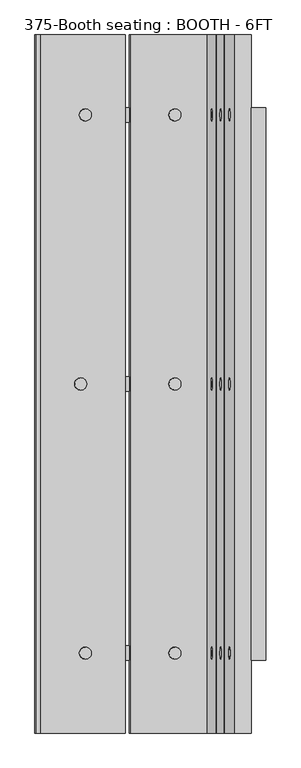
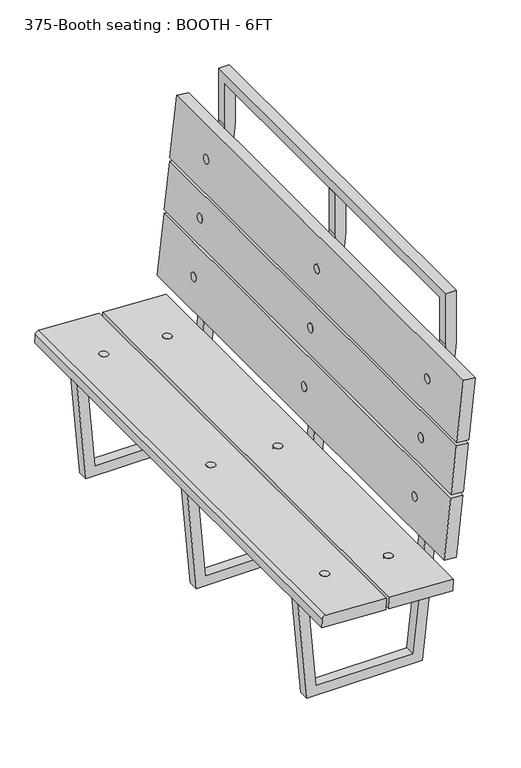
"""IFC4 building model written with IfcOpenShell, lengths in millimetres: furniture geometry, 375-Booth seating : BOOTH - 6FT."""

from ifc_helpers import new_model, si_unit, point, frame, frame_2d, origin, place, context, project, spatial, polyline, circle_curve, trimmed, segment, composite_curve, outline, extrude, faceted_brep, source, transform, mapped, element, save


def furniture_375_booth_seating_booth_6ft_239d0368(model_context):
    return source(origin(), model_context, "Body", "SolidModel", [
        extrude(outline(composite_curve([segment(trimmed(circle_curve(frame_2d((0.0, 15.875)), 15.875), [point((0.0, 31.75))], [point((0.0, 0.0))], False, "CARTESIAN"), True, "CONTINUOUS"), segment(trimmed(circle_curve(frame_2d((0.0, 15.875)), 15.875), [point((0.0, 0.0))], [point((0.0, 31.75))], False, "CARTESIAN"), True, "CONTINUOUS")], self_intersect=False)), frame((476.8022404, -688.975, 403.0070028), z_axis=(0.052335956242943765, 0.0, 0.9986295347545739), x_axis=(-0.9986295347545739, 0.0, 0.052335956242943765)), (0.0, 0.0, 1.0), 44.45),
        extrude(outline(composite_curve([segment(trimmed(circle_curve(frame_2d((-234.95, 15.875)), 15.875), [point((-234.95, 31.75))], [point((-234.95, 0.0))], False, "CARTESIAN"), True, "CONTINUOUS"), segment(trimmed(circle_curve(frame_2d((-234.95, 15.875)), 15.875), [point((-234.95, 0.0))], [point((-234.95, 31.75))], False, "CARTESIAN"), True, "CONTINUOUS")], self_intersect=False)), frame((476.8022404, -688.975, 403.0070028), z_axis=(0.052335956242943765, 0.0, 0.9986295347545739), x_axis=(-0.9986295347545739, 0.0, 0.052335956242943765)), (0.0, 0.0, 1.0), 44.45),
        extrude(outline(composite_curve([segment(trimmed(circle_curve(frame_2d((0.0, -1393.825)), 15.875), [point((0.0, -1377.95))], [point((0.0, -1409.7))], False, "CARTESIAN"), True, "CONTINUOUS"), segment(trimmed(circle_curve(frame_2d((0.0, -1393.825)), 15.875), [point((0.0, -1409.7))], [point((0.0, -1377.95))], False, "CARTESIAN"), True, "CONTINUOUS")], self_intersect=False)), frame((476.8022404, -688.975, 403.0070028), z_axis=(0.052335956242943765, 0.0, 0.9986295347545739), x_axis=(-0.9986295347545739, 0.0, 0.052335956242943765)), (0.0, 0.0, 1.0), 44.45),
        extrude(outline(composite_curve([segment(trimmed(circle_curve(frame_2d((-234.95, -1393.825)), 15.875), [point((-234.95, -1377.95))], [point((-234.95, -1409.7))], False, "CARTESIAN"), True, "CONTINUOUS"), segment(trimmed(circle_curve(frame_2d((-234.95, -1393.825)), 15.875), [point((-234.95, -1409.7))], [point((-234.95, -1377.95))], False, "CARTESIAN"), True, "CONTINUOUS")], self_intersect=False)), frame((476.8022404, -688.975, 403.0070028), z_axis=(0.052335956242943765, 0.0, 0.9986295347545739), x_axis=(-0.9986295347545739, 0.0, 0.052335956242943765)), (0.0, 0.0, 1.0), 44.45),
        extrude(outline(composite_curve([segment(trimmed(circle_curve(frame_2d((0.0, 15.875)), 15.875), [point((0.0, 31.75))], [point((0.0, 0.0))], False, "CARTESIAN"), True, "CONTINUOUS"), segment(trimmed(circle_curve(frame_2d((0.0, 15.875)), 15.875), [point((0.0, 0.0))], [point((0.0, 31.75))], False, "CARTESIAN"), True, "CONTINUOUS")], self_intersect=False)), frame((900.6975371, 720.725, 1069.1522612), z_axis=(-0.9945218953682735, 0.0, 0.10452846326765225), x_axis=(-0.10452846326765225, 0.0, -0.9945218953682735)), (0.0, 0.0, 1.0), 44.45),
        extrude(outline(composite_curve([segment(trimmed(circle_curve(frame_2d((222.2499999, 15.875)), 15.875), [point((222.2499999, 31.75))], [point((222.2499999, 0.0))], False, "CARTESIAN"), True, "CONTINUOUS"), segment(trimmed(circle_curve(frame_2d((222.2499999, 15.875)), 15.875), [point((222.2499999, 0.0))], [point((222.2499999, 31.75))], False, "CARTESIAN"), True, "CONTINUOUS")], self_intersect=False)), frame((900.6975371, 720.725, 1069.1522612), z_axis=(-0.9945218953682735, 0.0, 0.10452846326765225), x_axis=(-0.10452846326765225, 0.0, -0.9945218953682735)), (0.0, 0.0, 1.0), 44.45),
        extrude(outline(composite_curve([segment(trimmed(circle_curve(frame_2d((444.5, 15.875)), 15.875), [point((444.5, 31.75))], [point((444.5, 0.0))], False, "CARTESIAN"), True, "CONTINUOUS"), segment(trimmed(circle_curve(frame_2d((444.5, 15.875)), 15.875), [point((444.5, 0.0))], [point((444.5, 31.75))], False, "CARTESIAN"), True, "CONTINUOUS")], self_intersect=False)), frame((900.6975371, 720.725, 1069.1522612), z_axis=(-0.9945218953682735, 0.0, 0.10452846326765225), x_axis=(-0.10452846326765225, 0.0, -0.9945218953682735)), (0.0, 0.0, 1.0), 44.45),
        extrude(outline(composite_curve([segment(trimmed(circle_curve(frame_2d((0.0, 1425.575)), 15.875), [point((0.0, 1441.45))], [point((0.0, 1409.7))], False, "CARTESIAN"), True, "CONTINUOUS"), segment(trimmed(circle_curve(frame_2d((0.0, 1425.575)), 15.875), [point((0.0, 1409.7))], [point((0.0, 1441.45))], False, "CARTESIAN"), True, "CONTINUOUS")], self_intersect=False)), frame((900.6975371, 720.725, 1069.1522612), z_axis=(-0.9945218953682735, 0.0, 0.10452846326765225), x_axis=(-0.10452846326765225, 0.0, -0.9945218953682735)), (0.0, 0.0, 1.0), 44.45),
        extrude(outline(composite_curve([segment(trimmed(circle_curve(frame_2d((222.2499999, 1425.575)), 15.875), [point((222.2499999, 1441.45))], [point((222.2499999, 1409.7))], False, "CARTESIAN"), True, "CONTINUOUS"), segment(trimmed(circle_curve(frame_2d((222.2499999, 1425.575)), 15.875), [point((222.2499999, 1409.7))], [point((222.2499999, 1441.45))], False, "CARTESIAN"), True, "CONTINUOUS")], self_intersect=False)), frame((900.6975371, 720.725, 1069.1522612), z_axis=(-0.9945218953682735, 0.0, 0.10452846326765225), x_axis=(-0.10452846326765225, 0.0, -0.9945218953682735)), (0.0, 0.0, 1.0), 44.45),
        extrude(outline(composite_curve([segment(trimmed(circle_curve(frame_2d((444.5, 1425.575)), 15.875), [point((444.5, 1441.45))], [point((444.5, 1409.7))], False, "CARTESIAN"), True, "CONTINUOUS"), segment(trimmed(circle_curve(frame_2d((444.5, 1425.575)), 15.875), [point((444.5, 1409.7))], [point((444.5, 1441.45))], False, "CARTESIAN"), True, "CONTINUOUS")], self_intersect=False)), frame((900.6975371, 720.725, 1069.1522612), z_axis=(-0.9945218953682735, 0.0, 0.10452846326765225), x_axis=(-0.10452846326765225, 0.0, -0.9945218953682735)), (0.0, 0.0, 1.0), 44.45),
        extrude(outline(composite_curve([segment(trimmed(circle_curve(frame_2d((0.0, 15.875)), 15.875), [point((0.0, 31.75))], [point((0.0, 0.0))], False, "CARTESIAN"), True, "CONTINUOUS"), segment(trimmed(circle_curve(frame_2d((0.0, 15.875)), 15.875), [point((0.0, 0.0))], [point((0.0, 31.75))], False, "CARTESIAN"), True, "CONTINUOUS")], self_intersect=False)), frame((464.1196453, 15.875, 403.6716695), z_axis=(0.052335956242943765, 0.0, 0.9986295347545739), x_axis=(-0.9986295347545739, 0.0, 0.052335956242943765)), (0.0, 0.0, 1.0), 44.45),
        extrude(outline(composite_curve([segment(trimmed(circle_curve(frame_2d((-247.65, 15.875)), 15.875), [point((-247.65, 31.75))], [point((-247.65, 0.0))], False, "CARTESIAN"), True, "CONTINUOUS"), segment(trimmed(circle_curve(frame_2d((-247.65, 15.875)), 15.875), [point((-247.65, 0.0))], [point((-247.65, 31.75))], False, "CARTESIAN"), True, "CONTINUOUS")], self_intersect=False)), frame((464.1196453, 15.875, 403.6716695), z_axis=(0.052335956242943765, 0.0, 0.9986295347545739), x_axis=(-0.9986295347545739, 0.0, 0.052335956242943765)), (0.0, 0.0, 1.0), 44.45),
        extrude(outline(composite_curve([segment(trimmed(circle_curve(frame_2d((0.0, 15.875)), 15.875), [point((0.0, 31.75))], [point((0.0, 0.0))], False, "CARTESIAN"), True, "CONTINUOUS"), segment(trimmed(circle_curve(frame_2d((0.0, 15.875)), 15.875), [point((0.0, 0.0))], [point((0.0, 31.75))], False, "CARTESIAN"), True, "CONTINUOUS")], self_intersect=False)), frame((900.6975371, 15.875, 1069.1522612), z_axis=(-0.9945218953682735, 0.0, 0.10452846326765225), x_axis=(-0.10452846326765225, 0.0, -0.9945218953682735)), (0.0, 0.0, 1.0), 44.45),
        extrude(outline(composite_curve([segment(trimmed(circle_curve(frame_2d((222.2499999, 15.875)), 15.875), [point((222.2499999, 31.75))], [point((222.2499999, 0.0))], False, "CARTESIAN"), True, "CONTINUOUS"), segment(trimmed(circle_curve(frame_2d((222.2499999, 15.875)), 15.875), [point((222.2499999, 0.0))], [point((222.2499999, 31.75))], False, "CARTESIAN"), True, "CONTINUOUS")], self_intersect=False)), frame((900.6975371, 15.875, 1069.1522612), z_axis=(-0.9945218953682735, 0.0, 0.10452846326765225), x_axis=(-0.10452846326765225, 0.0, -0.9945218953682735)), (0.0, 0.0, 1.0), 44.45),
        extrude(outline(composite_curve([segment(trimmed(circle_curve(frame_2d((444.5, 15.875)), 15.875), [point((444.5, 31.75))], [point((444.5, 0.0))], False, "CARTESIAN"), True, "CONTINUOUS"), segment(trimmed(circle_curve(frame_2d((444.5, 15.875)), 15.875), [point((444.5, 0.0))], [point((444.5, 31.75))], False, "CARTESIAN"), True, "CONTINUOUS")], self_intersect=False)), frame((900.6975371, 15.875, 1069.1522612), z_axis=(-0.9945218953682735, 0.0, 0.10452846326765225), x_axis=(-0.10452846326765225, 0.0, -0.9945218953682735)), (0.0, 0.0, 1.0), 44.45),
        extrude(outline(polyline([(384.5625035, 828.7442542), (408.7701083, 366.8356381), (0.0, 402.5983885), (0.0, 826.6349718), (1193.8, 952.1084079), (1358.9, 952.1084079), (1358.9, 914.0084079), (1195.7967364, 914.0084079), (384.5625035, 828.7442542)]), holes=[polyline([(38.1, 437.5106063), (368.4284885, 408.6106083), (346.6192193, 824.7562543), (38.1, 792.3295777), (38.1, 437.5106063)])]), frame((0.0, -19.05, 0.0), z_axis=(0.0, 1.0, 0.0), x_axis=(0.0, 0.0, 1.0)), (0.0, 0.0, 1.0), 38.1),
        faceted_brep([(828.7442542, 685.8, 384.5625035), (366.8356381, 685.8, 408.7701083), (402.5983885, 685.8, 0.0), (826.6349718, 685.8, 0.0), (952.1084079, 685.8, 1193.8), (952.1084079, 685.8, 1358.9), (914.0084079, 685.8, 1358.9), (914.0084079, 685.8, 1195.7967364), (437.5106063, 685.8, 38.1), (408.6106083, 685.8, 368.4284885), (824.7562543, 685.8, 346.6192193), (792.3295777, 685.8, 38.1), (828.7442542, 723.9, 384.5625035), (914.0084079, 723.9, 1195.7967364), (914.0084079, 723.9, 1397.0), (952.1084079, 723.9, 1397.0), (952.1084079, 723.9, 1193.8), (826.6349718, 723.9, 0.0), (402.5983885, 723.9, 0.0), (366.8356381, 723.9, 408.7701083), (437.5106063, 723.9, 38.1), (792.3295777, 723.9, 38.1), (824.7562543, 723.9, 346.6192193), (408.6106083, 723.9, 368.4284885), (952.1084079, -685.8, 1358.9), (914.0084079, -685.8, 1358.9), (828.7442542, -723.9, 384.5625035), (366.8356381, -723.9, 408.7701083), (402.5983885, -723.9, 0.0), (826.6349718, -723.9, 0.0), (952.1084079, -723.9, 1193.8), (952.1084079, -723.9, 1397.0), (914.0084079, -723.9, 1397.0), (914.0084079, -723.9, 1195.7967364), (437.5106063, -723.9, 38.1), (408.6106083, -723.9, 368.4284885), (824.7562543, -723.9, 346.6192193), (792.3295777, -723.9, 38.1), (828.7442542, -685.8, 384.5625035), (914.0084079, -685.8, 1195.7967364), (952.1084079, -685.8, 1193.8), (826.6349718, -685.8, 0.0), (402.5983885, -685.8, 0.0), (366.8356381, -685.8, 408.7701083), (437.5106063, -685.8, 38.1), (792.3295777, -685.8, 38.1), (824.7562543, -685.8, 346.6192193), (408.6106083, -685.8, 368.4284885)], [[[0, 1, 2, 3, 4, 5, 6, 7], [8, 9, 10, 11]], [[12, 13, 14, 15, 16, 17, 18, 19], [20, 21, 22, 23]], [[3, 17, 16, 4]], [[7, 13, 12, 0]], [[0, 12, 19, 1]], [[1, 19, 18, 2]], [[2, 18, 17, 3]], [[8, 20, 23, 9]], [[9, 23, 22, 10]], [[10, 22, 21, 11]], [[11, 21, 20, 8]], [[6, 5, 24, 25]], [[26, 27, 28, 29, 30, 31, 32, 33], [34, 35, 36, 37]], [[38, 39, 25, 24, 40, 41, 42, 43], [44, 45, 46, 47]], [[26, 38, 43, 27]], [[27, 43, 42, 28]], [[28, 42, 41, 29]], [[34, 44, 47, 35]], [[35, 47, 46, 36]], [[36, 46, 45, 37]], [[37, 45, 44, 34]], [[29, 41, 40, 30]], [[33, 39, 38, 26]], [[15, 31, 30, 40, 24, 5, 4, 16]], [[14, 32, 31, 15]], [[13, 7, 6, 25, 39, 33, 32, 14]]]),
        extrude(outline(polyline([(0.0, 44.45), (1828.8, 44.45), (1828.8, 0.0), (0.0, 0.0), (0.0, 44.45)])), frame((841.955154, -914.4, 510.2558191), z_axis=(0.10452846326765272, 0.0, 0.9945218953682734), x_axis=(0.0, 1.0, 0.0)), (0.0, 0.0, 1.0), 234.95),
        extrude(outline(polyline([(0.0, 44.45), (1828.8, 44.45), (1828.8, 0.0), (0.0, 0.0), (0.0, 44.45)])), frame((867.8416279, -914.4, 756.5491664), z_axis=(0.10452846326765385, 0.0, 0.9945218953682733), x_axis=(0.0, 1.0, 0.0)), (0.0, 0.0, 1.0), 184.15),
        extrude(outline(polyline([(0.0, 44.45), (1828.8, 44.45), (1828.8, 0.0), (0.0, 0.0), (0.0, 44.45)])), frame((888.4180559, -914.4, 952.3208015), z_axis=(0.10452846326765004, 0.0, 0.9945218953682737), x_axis=(0.0, 1.0, 0.0)), (0.0, 0.0, 1.0), 234.95),
        extrude(outline(composite_curve([segment(polyline([(441.9125858, 583.7599832), (453.5442521, 361.8145691)]), True, "CONTINUOUS"), segment(trimmed(circle_curve(frame_2d((440.861657, 361.1499024)), 12.7), [point((453.5442521, 361.8145691))], [point((441.5263237, 348.4673073))], False, "CARTESIAN"), True, "CONTINUOUS"), segment(polyline([(441.5263237, 348.4673073), (409.8198359, 346.8056407), (397.4995564, 581.8905778), (441.9125858, 583.7599832)]), True, "CONTINUOUS")], self_intersect=False)), frame((0.0, -914.4, 0.0), z_axis=(0.0, 1.0, 0.0), x_axis=(0.0, 0.0, 1.0)), (0.0, 0.0, 1.0), 1828.8),
        extrude(outline(polyline([(0.0, 234.95), (1828.8, 234.95), (1828.8, 0.0), (0.0, 0.0), (0.0, 234.95)])), frame((828.7442542, -914.4, 384.5625035), z_axis=(0.05233595624294369, 0.0, 0.9986295347545739), x_axis=(0.0, 1.0, 0.0)), (0.0, 0.0, 1.0), 44.45),
    ])


if __name__ == "__main__":
    model = new_model("IFC4")
    model_context = context("Model", 3, world=origin())
    ifc_project = project(units=[si_unit("LENGTHUNIT", "METRE", prefix="MILLI")], contexts=[model_context])
    site = spatial("IfcSite", under=ifc_project)
    building = spatial("IfcBuilding", under=site)
    placement = place(None, origin())
    furniture_375_booth_seating_booth_6ft_shape = furniture_375_booth_seating_booth_6ft_239d0368(model_context)
    element("IfcFurniture", 1, ObjectType="375-Booth seating : BOOTH - 6FT", at=placement, inside=building, context=model_context, shape_type="MappedRepresentation", body=[
        mapped(furniture_375_booth_seating_booth_6ft_shape, transform((0.0, 0.0, 0.0), x_axis=(1.0, 0.0, 0.0), y_axis=(0.0, 1.0, 0.0), z_axis=(0.0, 0.0, 1.0))),
    ])
    save(model, "model.ifc")

# Revit data of these elements
# Type "375-Booth seating : BOOTH - 6FT"
#   tube dim [instance default] = 0' - 1 1/2"
#   seat angle = 3.00°
#   radius of plug = 0' - 0 5/8"
#   plank width_2 = 0' - 7 1/4"
#   plank width_1 = 0' - 9 1/4"
#   plank depth = 0' - 1 3/4"
#   inset = 0' - 9"
#   gap = 0' - 0 1/2"
#   DEPTH = 6' - 0"
#   Seating Count = 3
#   middle support visibility = yes
#   Right Bench Visible [instance default] = yes
#   Left Bench Visible [instance default] = yes
#   Material_1 = WOOD-OAKFIRE
#   Material 2 = 1 1/2" SQUARE TUBE STEEL\n- WELDED MITER JOINTS GROUND SMOOTH\n- CLEAR COAT
#   Assembly Code = ""
# Element 1 (IfcFurniture, "375-Booth seating : BOOTH - 6FT")
#   Materials on its faces: "1 1/2\" SQUARE TUBE STEEL\n- WELDED MITER JOINTS GROUND SMOOTH\n- CLEAR COAT", "1 1/4\" WOOD PLUG\n(SLIGHTLY DARKER OR STAINED WOOD) - GAL. HEX HEAD THRU BOLT", "WOOD-OAKFIRE"
# Materials
#   "WOOD-OAKFIRE": class "Wood", colour RGB 198 202 183, transparency 0, Description = "Generic wood", Cost = 0
#   "1 1/2\" SQUARE TUBE STEEL\n- WELDED MITER JOINTS GROUND SMOOTH\n- CLEAR COAT": class "Metal", colour RGB 147 147 147, transparency 0, Cost = 0
#   "1 1/4\" WOOD PLUG\n(SLIGHTLY DARKER OR STAINED WOOD) - GAL. HEX HEAD THRU BOLT": class "Generic", colour RGB 192 192 192, transparency 0, Cost = 0
